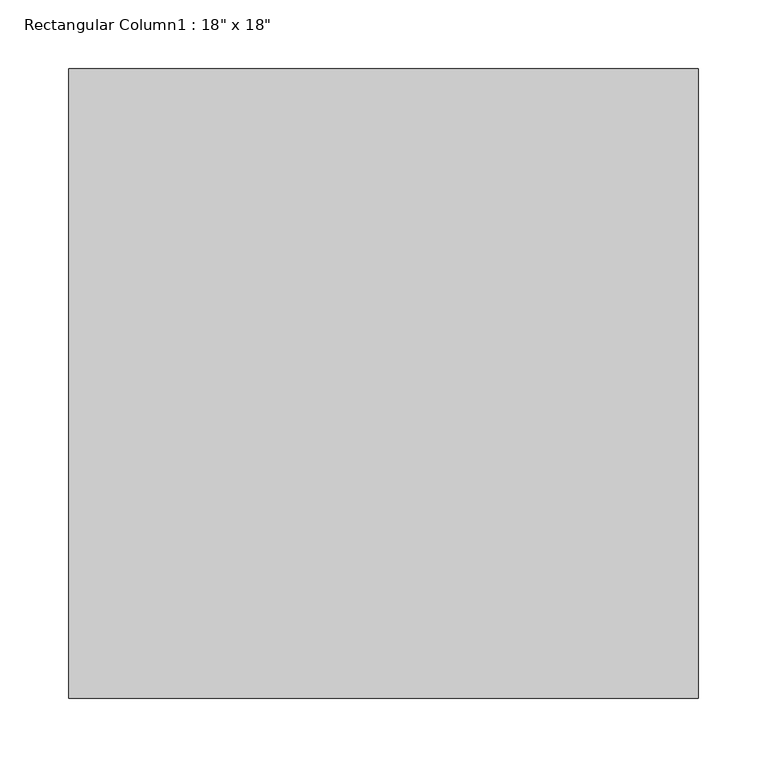
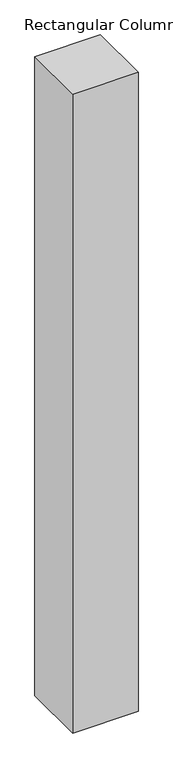
"""IFC4 building model written with IfcOpenShell, lengths in millimetres: column geometry."""

from ifc_helpers import new_model, si_unit, frame, origin, place, context, project, spatial, polyline, outline, extrude, source, transform, mapped, element, save


def column_2b57f2af(model_context):
    return source(origin(), model_context, "Body", "SweptSolid", [
        extrude(outline(polyline([(228.6, 228.6), (228.6, -228.6), (-228.6, -228.6), (-228.6, 228.6), (228.6, 228.6)])), frame((0.0, 0.0, 10210.8), z_axis=(0.0, 0.0, 1.0), x_axis=(1.0, 0.0, 0.0)), (0.0, 0.0, 1.0), 4724.4),
    ])


if __name__ == "__main__":
    model = new_model("IFC4")
    model_context = context("Model", 3, world=origin())
    ifc_project = project(units=[si_unit("LENGTHUNIT", "METRE", prefix="MILLI")], contexts=[model_context])
    site = spatial("IfcSite", under=ifc_project)
    building = spatial("IfcBuilding", under=site)
    placement = place(None, origin())
    column_shape = column_2b57f2af(model_context)
    element("IfcColumn", 1, ObjectType="Rectangular Column1 : 18\" x 18\"", at=placement, inside=building, context=model_context, shape_type="MappedRepresentation", body=[
        mapped(column_shape, transform((0.0, 0.0, 0.0), x_axis=(1.0, 0.0, 0.0), y_axis=(0.0, 1.0, 0.0), z_axis=(0.0, 0.0, 1.0))),
    ])
    save(model, "model.ifc")

# Revit data of these elements
# Type "Rectangular Column1 : 18\" x 18\""
#   Depth = 1' - 6"
#   Width = 1' - 6"
